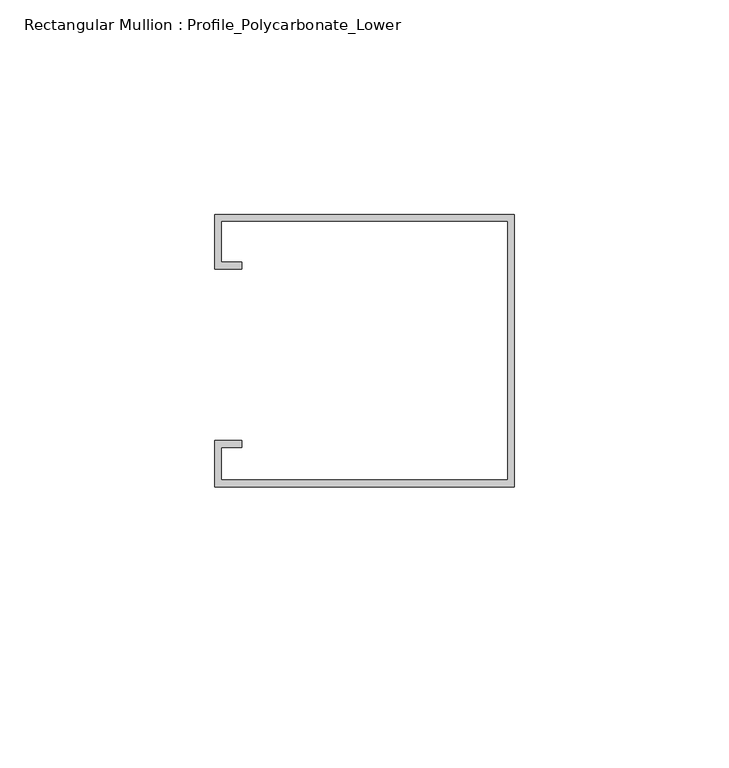
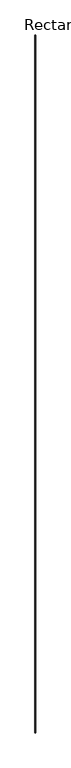
"""IFC4 building model written with IfcOpenShell, lengths in millimetres: member geometry, Rectangular Mullion : Profile_Polycarbonate_Lower."""

from ifc_helpers import new_model, si_unit, frame, origin, place, context, project, spatial, polyline, outline, extrude, source, transform, mapped, element, save


def rectangular_mullion_profile_polycarbonate_lower_eeddcbd2(model_context):
    return source(origin(), model_context, "Body", "SweptSolid", [
        extrude(outline(polyline([(0.0, 32.7), (0.0, -30.8), (-69.85, -30.8), (-69.85, -20.0), (-63.5, -20.0), (-63.5, -21.5875), (-68.2625, -21.5875), (-68.2625, -29.2125), (-1.5875, -29.2125), (-1.5875, 31.1125), (-68.2625, 31.1125), (-68.2625, 21.5875), (-63.5, 21.5875), (-63.5, 20.0), (-69.85, 20.0), (-69.85, 32.7), (0.0, 32.7)])), frame((0.0, 0.0, -88538.05), z_axis=(0.0, 0.0, 1.0), x_axis=(1.0, 0.0, 0.0)), (0.0, 0.0, 1.0), 88538.05),
    ])


if __name__ == "__main__":
    model = new_model("IFC4")
    model_context = context("Model", 3, world=origin())
    ifc_project = project(units=[si_unit("LENGTHUNIT", "METRE", prefix="MILLI")], contexts=[model_context])
    site = spatial("IfcSite", under=ifc_project)
    building = spatial("IfcBuilding", under=site)
    placement = place(None, origin())
    rectangular_mullion_profile_polycarbonate_lower_shape = rectangular_mullion_profile_polycarbonate_lower_eeddcbd2(model_context)
    element("IfcMember", 1, ObjectType="Rectangular Mullion : Profile_Polycarbonate_Lower", at=placement, inside=building, context=model_context, shape_type="MappedRepresentation", body=[
        mapped(rectangular_mullion_profile_polycarbonate_lower_shape, transform((0.0, 0.0, 0.0), x_axis=(1.0, 0.0, 0.0), y_axis=(0.0, 1.0, 0.0), z_axis=(0.0, 0.0, 1.0))),
    ])
    save(model, "model.ifc")

# Revit data of these elements
# Type "Rectangular Mullion : Profile_Polycarbonate_Lower"
#   built-in parameter 1007322 = 0.208333 (stored number, unit not read)
#   built-in parameter 1007321 = 0 (stored number, unit not read)
#   built-in parameter 1007320 = 0.00520833 (stored number, unit not read)
